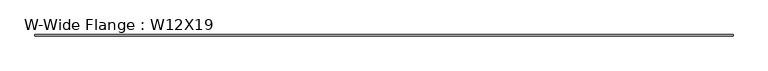
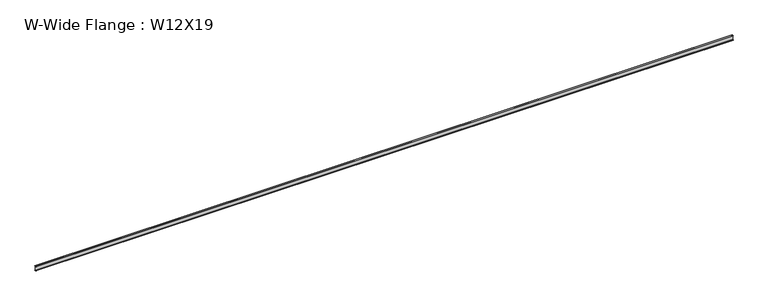
"""IFC4 building model written with IfcOpenShell, lengths in millimetres: beam geometry, W-Wide Flange : W12X19."""

from ifc_helpers import new_model, si_unit, point, frame, frame_2d, origin, place, context, project, spatial, polyline, circle_curve, trimmed, segment, composite_curve, outline, extrude, source, transform, mapped, element, save


def w_wide_flange_w12x19_2a407e1f(model_context):
    return source(origin(), model_context, "Body", "SweptSolid", [
        extrude(outline(composite_curve([segment(polyline([(50.927, -146.05), (50.927, -154.94), (-50.927, -154.94), (-50.927, -146.05), (-16.3195, -146.05)]), True, "CONTINUOUS"), segment(trimmed(circle_curve(frame_2d((-16.3195, -132.715)), 13.335), [point((-16.3195, -146.05))], [point((-2.9845, -132.715))], True, "CARTESIAN"), True, "CONTINUOUS"), segment(polyline([(-2.9845, -132.715), (-2.9845, 132.715)]), True, "CONTINUOUS"), segment(trimmed(circle_curve(frame_2d((-16.3195, 132.715)), 13.335), [point((-2.9845, 132.715))], [point((-16.3195, 146.05))], True, "CARTESIAN"), True, "CONTINUOUS"), segment(polyline([(-16.3195, 146.05), (-50.927, 146.05), (-50.927, 154.94), (50.927, 154.94), (50.927, 146.05), (16.3195, 146.05)]), True, "CONTINUOUS"), segment(trimmed(circle_curve(frame_2d((16.3195, 132.715)), 13.335), [point((16.3195, 146.05))], [point((2.9845, 132.715))], True, "CARTESIAN"), True, "CONTINUOUS"), segment(polyline([(2.9845, 132.715), (2.9845, -132.715)]), True, "CONTINUOUS"), segment(trimmed(circle_curve(frame_2d((16.3195, -132.715)), 13.335), [point((2.9845, -132.715))], [point((16.3195, -146.05))], True, "CARTESIAN"), True, "CONTINUOUS"), segment(polyline([(16.3195, -146.05), (50.927, -146.05)]), True, "CONTINUOUS")], self_intersect=False)), frame((-23771.225, 0.0, 0.0), z_axis=(1.0, 0.0, 0.0), x_axis=(0.0, 1.0, 0.0)), (0.0, 0.0, 1.0), 47517.05),
    ])


if __name__ == "__main__":
    model = new_model("IFC4")
    model_context = context("Model", 3, world=origin())
    ifc_project = project(units=[si_unit("LENGTHUNIT", "METRE", prefix="MILLI")], contexts=[model_context])
    site = spatial("IfcSite", under=ifc_project)
    building = spatial("IfcBuilding", under=site)
    placement = place(None, origin())
    w_wide_flange_w12x19_shape = w_wide_flange_w12x19_2a407e1f(model_context)
    element("IfcBeam", 1, ObjectType="W-Wide Flange : W12X19", at=placement, inside=building, context=model_context, shape_type="MappedRepresentation", body=[
        mapped(w_wide_flange_w12x19_shape, transform((0.0, 0.0, 0.0), x_axis=(1.0, 0.0, 0.0), y_axis=(0.0, 1.0, 0.0), z_axis=(0.0, 0.0, 1.0))),
    ])
    save(model, "model.ifc")

# Revit data of these elements
# Type "W-Wide Flange : W12X19"
#   Assembly Code = "B10"
#   W = 19
#   Length [instance default] = 5' - 0"
#   bf = 0' - 4.01"
#   d = 1' - 0.2"
#   k = 0' - 0 7/8"
#   k2 = 0' - 0.525"
#   tf = 0' - 0.35"
#   tw = 0' - 0.235"
#   A = 0.0386806 SF
#   Structural Material [instance default] = Steel ASTM A992
# Element 1 (IfcBeam, "W-Wide Flange : W12X19")
#   Structural Material = STRUCTURAL STEEL - SEE STRUCT. DWGS
#   Materials on its faces: "STRUCTURAL STEEL - SEE STRUCT. DWGS"
# Materials
#   "Steel ASTM A992": class "Metal", colour RGB 199 199 199, transparency 0, Description = "Structural steel 50ksi", Cost = 0
#   "STRUCTURAL STEEL - SEE STRUCT. DWGS": class "Metal", colour RGB 137 146 153, transparency 0, Description = "Steel, mill finish", Cost = 0
